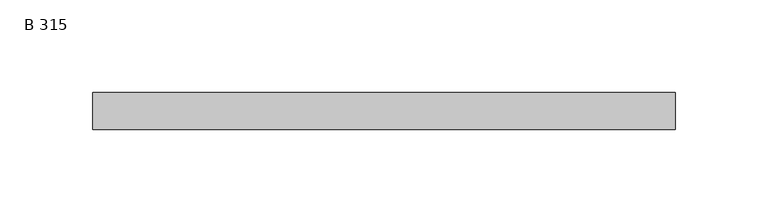
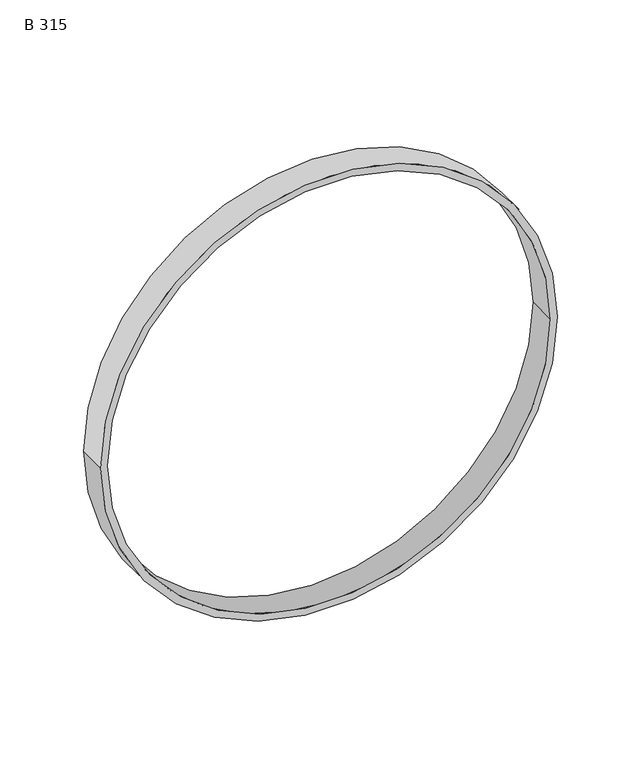
"""IFC4 building model written with IfcOpenShell, lengths in millimetres: proxy geometry, Гибкая вставка B : B 315."""

from ifc_helpers import new_model, si_unit, point, frame, origin, origin_2d, place, context, project, spatial, circle_curve, trimmed, segment, composite_curve, outline, extrude, source, transform, mapped, element, save


def b_315_c0d1b37d(model_context):
    return source(origin(), model_context, "Body", "SweptSolid", [
        extrude(outline(composite_curve([segment(trimmed(circle_curve(origin_2d(), 157.5), [point((0.0, -157.5))], [point((0.0, 157.5))], False, "CARTESIAN"), True, "CONTINUOUS"), segment(trimmed(circle_curve(origin_2d(), 157.5), [point((0.0, 157.5))], [point((0.0, -157.5))], False, "CARTESIAN"), True, "CONTINUOUS")], self_intersect=False), holes=[composite_curve([segment(trimmed(circle_curve(origin_2d(), 152.5), [point((0.0, -152.5))], [point((0.0, 152.5))], True, "CARTESIAN"), True, "CONTINUOUS"), segment(trimmed(circle_curve(origin_2d(), 152.5), [point((0.0, 152.5))], [point((0.0, -152.5))], True, "CARTESIAN"), True, "CONTINUOUS")], self_intersect=False)]), frame((0.0, -10.0, 0.0), z_axis=(0.0, 1.0, 0.0), x_axis=(0.0, 0.0, 1.0)), (0.0, 0.0, 1.0), 20.0),
    ])


if __name__ == "__main__":
    model = new_model("IFC4")
    model_context = context("Model", 3, world=origin())
    ifc_project = project(units=[si_unit("LENGTHUNIT", "METRE", prefix="MILLI")], contexts=[model_context])
    site = spatial("IfcSite", under=ifc_project)
    building = spatial("IfcBuilding", under=site)
    placement = place(None, origin())
    b_315_shape = b_315_c0d1b37d(model_context)
    element("IfcBuildingElementProxy", 1, Name="Гибкая вставка B : B 315", ObjectType="Гибкая вставка B : B 315", at=placement, inside=building, context=model_context, shape_type="MappedRepresentation", body=[
        mapped(b_315_shape, transform((0.0, 0.0, 0.0), x_axis=(1.0, 0.0, 0.0), y_axis=(0.0, 1.0, 0.0), z_axis=(0.0, 0.0, 1.0))),
    ])
    save(model, "model.ifc")

# Revit data of these elements
# Type "Гибкая вставка B : B 315"
#   ADSK_Система_Имя [instance default] = ""
#   ADSK_Наименование краткое = "B 315"
#   ADSK_Наименование [instance default] = "Гибкая вставка B 315"
#   ADSK_Масса_Текст = ""
#   ADSK_Марка = ""
#   ADSK_Код изделия = ""
#   ADSK_Завод-изготовитель = "WAER"
#   ADSK_Единица измерения = "шт."
#   ADSK_URL страницы изделия = ""
#   ADSK_URL документации изделия = ""
#   ADSK_Расход воздуха = 0 m³/h
#   ADSK_Размер_Длина_L = 20 mm
#   ADSK_Размер_Диаметр_D1 = 305 mm
#   ADSK_Размер_Диаметр_D = 315 mm
#   ADSK_Потеря давления воздуха = 0.0 Pa
#   ADSK_Масса = 0
#   ADSK_Количество [instance default] = 1
#   Default Elevation = 0
#   URL = ""
#   Cost = 0
